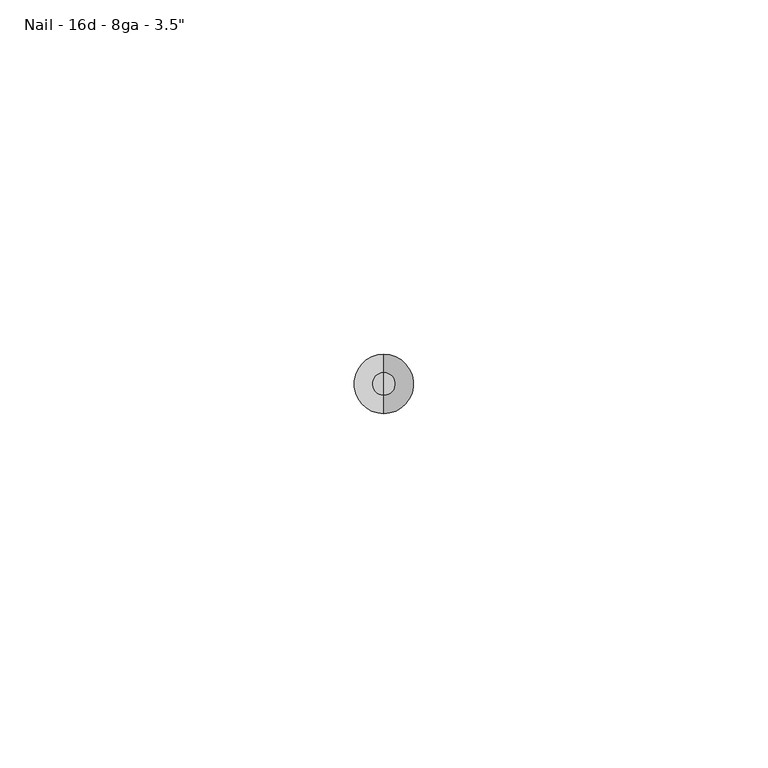
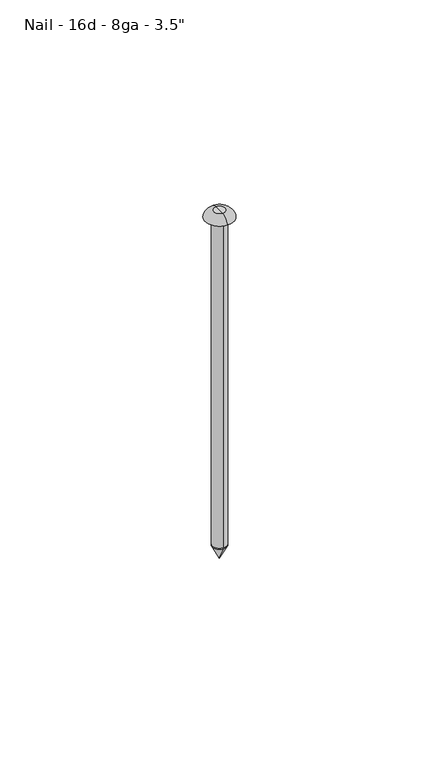
"""IFC4 building model written with IfcOpenShell, lengths in millimetres: fastener geometry."""

from ifc_helpers import new_model, si_unit, point, frame, origin, origin_2d, place, context, project, spatial, polyline, circle_curve, ellipse_curve, trimmed, segment, composite_curve, outline, extrude, source, transform, mapped, element, save
from ifc_brep_helpers import plane_surface, revolved_surface, advanced_brep


def fastener_01815b45(model_context):
    return source(origin(), model_context, "Body", "SolidModel", [
        advanced_brep(
        [(0.0, -2.0955, -101.6), (0.0, 2.0955, -101.6), (0.0, 0.0, -101.6), (0.0, 0.0, -105.791)],
        [
            (0, 1, circle_curve(frame((0.0, 0.0, -101.6), z_axis=(0.0, 0.0, 1.0), x_axis=(0.0, 1.0, 0.0)), 2.0955)),
            (1, 2),
            (2, 0),
            (1, 0, circle_curve(frame((0.0, 0.0, -101.6), z_axis=(0.0, 0.0, 1.0), x_axis=(0.0, 1.0, 0.0)), 2.0955)),
            (3, 1),
            (0, 3),
        ],
        [
            plane_surface(frame((0.0, 0.0, -101.6), z_axis=(0.0, 0.0, 1.0), x_axis=(0.0, 1.0, 0.0))),
            revolved_surface(polyline([(0.0, 2.0955, -101.6), (0.0, 0.0, -105.791)]), (0.0, 0.0, -103.0840259), (0.0, 0.0, -1.0)),
        ],
        [
            (0, [[1, 2, 3]]),
            (0, [[4, -3, -2]]),
            (1, [[5, -1, 6]]),
            (1, [[-6, -4, -5]]),
        ],
    ),
        advanced_brep(
        [(0.0, 4.191, 0.0), (0.0, -4.191, 0.0), (0.0, 0.0, 0.0), (0.0, 0.0, 2.0955), (0.0, -1.5875, 2.0955), (0.0, 1.5875, 2.0955)],
        [
            (0, 1, circle_curve(frame((0.0, 0.0, 0.0), z_axis=(0.0, 0.0, -1.0), x_axis=(0.0, -1.0, 0.0)), 4.191)),
            (1, 2),
            (2, 0),
            (1, 0, circle_curve(frame((0.0, 0.0, 0.0), z_axis=(0.0, 0.0, -1.0), x_axis=(0.0, -1.0, 0.0)), 4.191)),
            (3, 4),
            (4, 5, circle_curve(frame((0.0, 0.0, 2.0955), z_axis=(0.0, 0.0, 1.0), x_axis=(0.0, -1.0, 0.0)), 1.5875)),
            (5, 3),
            (5, 4, circle_curve(frame((0.0, 0.0, 2.0955), z_axis=(0.0, 0.0, 1.0), x_axis=(0.0, -1.0, 0.0)), 1.5875)),
            (4, 1, circle_curve(frame((0.0, -1.5875, -0.5695758), z_axis=(1.0, 0.0, 0.0), x_axis=(0.0, -1.0, 0.0)), 2.6650758)),
            (0, 5, circle_curve(frame((0.0, 1.5875, -0.5695758), z_axis=(1.0, 0.0, 0.0), x_axis=(0.0, 1.0, 0.0)), 2.6650758)),
        ],
        [
            plane_surface(frame((0.0, 0.0, 0.0), z_axis=(0.0, 0.0, -1.0), x_axis=(0.0, -1.0, 0.0))),
            plane_surface(frame((0.0, 0.0, 2.0955), z_axis=(0.0, 0.0, 1.0), x_axis=(0.0, -1.0, 0.0))),
            revolved_surface(trimmed(ellipse_curve(frame((0.0, -1.5875, -0.5695758), z_axis=(-1.0, 0.0, 0.0), x_axis=(0.0, -1.0, 0.0)), 2.6650758, 2.6650758), [point((0.0, -4.191, 0.0))], [point((0.0, -1.5875, 2.0955))], True, "CARTESIAN"), (0.0, 0.0, 1.4840259), (0.0, 0.0, 1.0)),
        ],
        [
            (0, [[1, 2, 3]]),
            (0, [[4, -3, -2]]),
            (1, [[5, 6, 7]]),
            (1, [[-7, 8, -5]]),
            (2, [[-6, 9, -1, 10]]),
            (2, [[-8, -10, -4, -9]]),
        ],
    ),
        extrude(outline(composite_curve([segment(trimmed(circle_curve(origin_2d(), 2.0955), [point((0.0, -2.0955))], [point((0.0, 2.0955))], False, "CARTESIAN"), True, "CONTINUOUS"), segment(trimmed(circle_curve(origin_2d(), 2.0955), [point((0.0, 2.0955))], [point((0.0, -2.0955))], False, "CARTESIAN"), True, "CONTINUOUS")], self_intersect=False)), frame((0.0, 0.0, -101.6), z_axis=(0.0, 0.0, 1.0), x_axis=(1.0, 0.0, 0.0)), (0.0, 0.0, 1.0), 101.6),
    ])


if __name__ == "__main__":
    model = new_model("IFC4")
    model_context = context("Model", 3, world=origin())
    ifc_project = project(units=[si_unit("LENGTHUNIT", "METRE", prefix="MILLI")], contexts=[model_context])
    site = spatial("IfcSite", under=ifc_project)
    building = spatial("IfcBuilding", under=site)
    placement = place(None, origin())
    fastener_shape = fastener_01815b45(model_context)
    element("IfcFastener", 1, ObjectType="060523 - W_P_C - Fastenings - Generic : Nail - 16d - 8ga - 3.5\"", at=placement, inside=building, context=model_context, shape_type="MappedRepresentation", body=[
        mapped(fastener_shape, transform((0.0, 0.0, 0.0), x_axis=(1.0, 0.0, 0.0), y_axis=(0.0, 1.0, 0.0), z_axis=(0.0, 0.0, 1.0))),
    ])
    save(model, "model.ifc")

# Revit data of these elements
# Project information
#   Project Issue Date = "Issue Date"
#   Project Status = "Project Status"
#   Client Name = "Owner"
#   Project Address = "Enter address here"
#   Project Name = "Project Name"
#   Project Number = "Project Number"
# Type "060523 - W_P_C - Fastenings - Generic : Nail - 16d - 8ga - 3.5\""
#   Washer_Thickness = 0' - 0.00333"
#   Washer Radius = 0' - 0.0925"
#   Washer Offset - Head = 0' - 0"
#   Washer Offset = 0' - 0"
#   Thickness_of_Substrate [instance default] = 0' - 1"
#   Side = 0' - 0 37/64"
#   Radius = 0' - 0.0825"
#   Length [instance default] = 0' - 3 1/2"
#   Head Size = 0' - 1"
#   Head Radius = 0' - 0 1/2"
#   Head Height = 0' - 0.01"
#   Double Diameter = 0' - 0.33"
#   Diameter = 0' - 0.165"
#   Default Elevation = 4' - 0"
#   Washer_Nut_Visibility = no
#   Washer_Head_Visibility = no
#   Round_Head_Visibility = yes
#   Point Visibility = yes
#   Nut_Visibility = no
#   Hex_Head_Visiblilty = no
#   Washer Material = none
#   Bolt Material (Size) = AT SILL - FASTENER AT 24" O.C.
# Element 1 (IfcFastener, "060523 - W_P_C - Fastenings - Generic : Nail - 16d - 8ga - 3.5\"")
#   Length = 0' - 4"
#   Materials on its faces: "AT SILL - FASTENER AT 24\" O.C."
# Materials
#   "AT SILL - FASTENER AT 24\" O.C.": class "Generic", colour RGB 120 120 120, transparency 0, Cost = 0
